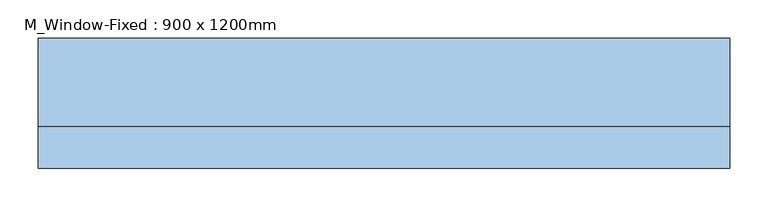
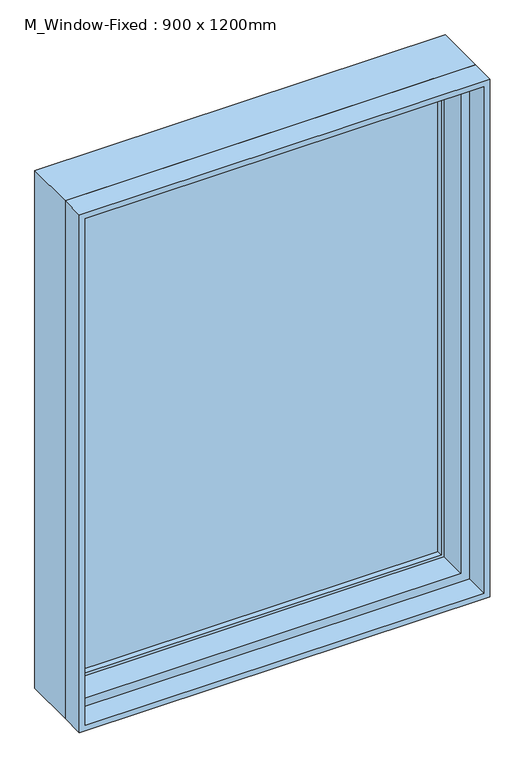
"""IFC4 building model written with IfcOpenShell, lengths in millimetres: window geometry, M_Window-Fixed : 900 x 1200mm."""

import ifcopenshell
import ifcopenshell.guid

model = None  # the IFC model being written
_history = None  # IfcOwnerHistory: only IFC2X3 demands one
_inside = {}  # id of a spatial element -> (the spatial element, [elements in it])
_under = {}  # id of a project, library or spatial element -> (it, [spatial elements below it])
_declared = {}  # id of a project -> (the project, [libraries it declares])
_typed = {}  # id of a type object -> (the type object, [elements of that type])
_made_of = {}  # id of a material, layer set ... -> (it, [elements and type objects made of it])


def new_model(schema):
    """Start an empty IFC model of exactly this schema.

    Asked for "IFC4X3", IfcOpenShell would pick the latest addendum, in which some entities
    have other attributes; the version numbers below select the first issue.
    IFC2X3 requires an IfcOwnerHistory on every rooted entity: one is made here for all.
    """
    global model, _history
    if schema == "IFC4X3":
        model = ifcopenshell.file(schema_version=(4, 3, 0, 0))
    else:
        model = ifcopenshell.file(schema=schema)
    _inside.clear()
    _under.clear()
    _declared.clear()
    _typed.clear()
    _made_of.clear()
    _history = None
    if model.schema == "IFC2X3":
        org = make("IfcOrganization", Name="unknown")
        user = make(
            "IfcPersonAndOrganization",
            ThePerson=make("IfcPerson", FamilyName="unknown"),
            TheOrganization=org,
        )
        app = make(
            "IfcApplication",
            ApplicationDeveloper=org,
            Version="unknown",
            ApplicationFullName="unknown",
            ApplicationIdentifier="unknown",
        )
        _history = make(
            "IfcOwnerHistory",
            OwningUser=user,
            OwningApplication=app,
            ChangeAction="ADDED",
            CreationDate=0,
        )
    return model


def make(cls, **values):
    """One entity of the class cls with the attributes given. An attribute that is None is left unset."""
    return model.create_entity(
        cls, **{name: value for name, value in values.items() if value is not None}
    )


def rooted(cls, **values):
    """An entity with a GlobalId (a new one), such as an element, a storey or a relation."""
    return make(cls, GlobalId=ifcopenshell.guid.new(), OwnerHistory=_history, **values)


def si_unit(unit_type, name, prefix=None):
    """IfcSIUnit, for example si_unit("LENGTHUNIT", "METRE", prefix="MILLI")."""
    return make("IfcSIUnit", UnitType=unit_type, Prefix=prefix, Name=name)


def assignment(units):
    """IfcUnitAssignment: the units of a project."""
    return None if units is None else make("IfcUnitAssignment", Units=units)


def point(xyz):
    """IfcCartesianPoint."""
    return None if xyz is None else make("IfcCartesianPoint", Coordinates=xyz)


def direction(xyz):
    """IfcDirection."""
    return None if xyz is None else make("IfcDirection", DirectionRatios=xyz)


def frame(location, z_axis=None, x_axis=None):
    """IfcAxis2Placement3D, a coordinate frame: its origin and axes. An axis left out is left unset."""
    return make(
        "IfcAxis2Placement3D",
        Location=point(location),
        Axis=direction(z_axis),
        RefDirection=direction(x_axis),
    )


def origin():
    """The frame at (0, 0, 0) with its axes left unset."""
    return frame((0.0, 0.0, 0.0))


def place(relative_to, where):
    """IfcLocalPlacement: puts the frame where relative to a parent placement (None: the world)."""
    return make(
        "IfcLocalPlacement", PlacementRelTo=relative_to, RelativePlacement=where
    )


def context(
    kind, dimensions, precision=None, world=None, true_north=None, identifier=None
):
    """IfcGeometricRepresentationContext, for example the 3D "Model" context."""
    return make(
        "IfcGeometricRepresentationContext",
        ContextIdentifier=identifier,
        ContextType=kind,
        CoordinateSpaceDimension=dimensions,
        Precision=precision,
        WorldCoordinateSystem=world,
        TrueNorth=true_north,
    )


def project(units=None, contexts=None):
    """IfcProject with its units and contexts."""
    return rooted(
        "IfcProject",
        Name="project",
        RepresentationContexts=contexts,
        UnitsInContext=assignment(units),
    )


def spatial(cls, under=None, at=None, **own):
    """A site, building, storey or space (cls), placed at a placement, below another one or the project."""
    s = rooted(cls, ObjectPlacement=at, **own)
    if under is not None:
        _under.setdefault(under.id(), (under, []))[1].append(s)
    return s


def polyline(points):
    """IfcPolyline through the points."""
    return make("IfcPolyline", Points=[point(p) for p in points])


def outline(outer, holes=None, kind="AREA"):
    """IfcArbitraryClosedProfileDef: a profile drawn as a closed curve; with holes, ...WithVoids."""
    if holes is None:
        return make("IfcArbitraryClosedProfileDef", ProfileType=kind, OuterCurve=outer)
    return make(
        "IfcArbitraryProfileDefWithVoids",
        ProfileType=kind,
        OuterCurve=outer,
        InnerCurves=holes,
    )


def extrude(swept, where, along, depth):
    """IfcExtrudedAreaSolid: the profile swept, set in the frame where, extruded along a direction by depth."""
    return make(
        "IfcExtrudedAreaSolid",
        SweptArea=swept,
        Position=where,
        ExtrudedDirection=direction(along),
        Depth=depth,
    )


def faces_of(points, faces, orient=None, outer=None):
    """IfcFace entities. A face is a list of loops; a loop is a list of indices into points, from 0.

    orient and outer hold one flag for each loop. By default every Orientation is true, the
    first loop of a face is its IfcFaceOuterBound and the others are IfcFaceBound.
    """
    made = []
    for i, loops in enumerate(faces):
        bounds = []
        for j, loop in enumerate(loops):
            is_outer = j == 0 if outer is None else outer[i][j]
            bounds.append(
                make(
                    "IfcFaceOuterBound" if is_outer else "IfcFaceBound",
                    Bound=make("IfcPolyLoop", Polygon=[points[k] for k in loop]),
                    Orientation=True if orient is None else orient[i][j],
                )
            )
        made.append(make("IfcFace", Bounds=bounds))
    return made


def faceted_brep(points, faces, orient=None, outer=None, voids=None):
    """IfcFacetedBrep: a solid bounded by flat faces; with voids (closed shells), ...WithVoids."""
    shared = [point(p) for p in points]
    hull = make("IfcClosedShell", CfsFaces=faces_of(shared, faces, orient, outer))
    if voids is None:
        return make("IfcFacetedBrep", Outer=hull)
    return make(
        "IfcFacetedBrepWithVoids",
        Outer=hull,
        Voids=[
            make(cls, CfsFaces=faces_of(shared, fs, o, b)) for cls, fs, o, b in voids
        ],
    )


def shape(context_of_items, identifier, shape_type, items):
    """IfcShapeRepresentation: the items that make up one representation, for example the "Body"."""
    return make(
        "IfcShapeRepresentation",
        ContextOfItems=context_of_items,
        RepresentationIdentifier=identifier,
        RepresentationType=shape_type,
        Items=items,
    )


def source(mapping_origin, context_of_items, identifier, shape_type, items):
    """IfcRepresentationMap: a shape defined once, which mapped items show again and again."""
    return make(
        "IfcRepresentationMap",
        MappingOrigin=mapping_origin,
        MappedRepresentation=shape(context_of_items, identifier, shape_type, items),
    )


def transform(
    local_origin,
    x_axis=None,
    y_axis=None,
    z_axis=None,
    scale=None,
    scale2=None,
    scale3=None,
    uniform=True,
):
    """IfcCartesianTransformationOperator3D, or its non-uniform kind. x_axis, y_axis, z_axis: its Axis1, 2, 3."""
    if uniform:
        return make(
            "IfcCartesianTransformationOperator3D",
            Axis1=direction(x_axis),
            Axis2=direction(y_axis),
            LocalOrigin=point(local_origin),
            Scale=scale,
            Axis3=direction(z_axis),
        )
    return make(
        "IfcCartesianTransformationOperator3DnonUniform",
        Axis1=direction(x_axis),
        Axis2=direction(y_axis),
        LocalOrigin=point(local_origin),
        Scale=scale,
        Axis3=direction(z_axis),
        Scale2=scale2,
        Scale3=scale3,
    )


def mapped(mapping_source, mapping_target):
    """IfcMappedItem: shows the shape of a source again, moved by a transform."""
    return make(
        "IfcMappedItem", MappingSource=mapping_source, MappingTarget=mapping_target
    )


def made_of(thing, what):
    """Note that an element or type object is made of a material, layer set ...; save() writes the relation."""
    if what is not None:
        _made_of.setdefault(what.id(), (what, []))[1].append(thing)
    return thing


def element(
    cls,
    number,
    at=None,
    inside=None,
    cuts=None,
    type_object=None,
    material=None,
    context=None,
    identifier="Body",
    shape_type=None,
    held_by="IfcProductDefinitionShape",
    body=None,
    shapes=None,
    **own,
):
    """One element of the class cls, such as IfcWall. Its Tag is "e" and its number.

    at: its placement. inside: the storey or other place that contains it. cuts: it is an
    opening in that element (IfcRelVoidsElement). A single representation is given by context,
    identifier, shape_type and body (its items); several are given by shapes. held_by: the class
    of the entity that holds the representations. save() writes the other relations.
    """
    e = rooted(cls, Tag="e%d" % number, ObjectPlacement=at, **own)
    if body is not None:
        shapes = [shape(context, identifier, shape_type, body)]
    if shapes is not None:
        e.Representation = make(held_by, Representations=shapes)
    if inside is not None:
        _inside.setdefault(inside.id(), (inside, []))[1].append(e)
    if cuts is not None:
        rooted(
            "IfcRelVoidsElement", RelatingBuildingElement=cuts, RelatedOpeningElement=e
        )
    if type_object is not None:
        _typed.setdefault(type_object.id(), (type_object, []))[1].append(e)
    return made_of(e, material)


def aggregate(whole, parts):
    """IfcRelAggregates: a whole, such as a stair, and the parts it consists of."""
    return rooted("IfcRelAggregates", RelatingObject=whole, RelatedObjects=parts)


def save(model, path):
    """Write the relations noted so far, then the file.

    IfcRelAggregates (storeys below a building ...), IfcRelContainedInSpatialStructure (elements
    in a storey), IfcRelDefinesByType, IfcRelAssociatesMaterial and IfcRelDeclares: one each for
    every whole, place, type object, material and project.
    """
    for whole, parts in _under.values():
        aggregate(whole, parts)
    for where, things in _inside.values():
        rooted(
            "IfcRelContainedInSpatialStructure",
            RelatedElements=things,
            RelatingStructure=where,
        )
    for kind, things in _typed.values():
        rooted("IfcRelDefinesByType", RelatedObjects=things, RelatingType=kind)
    for what, things in _made_of.values():
        rooted("IfcRelAssociatesMaterial", RelatedObjects=things, RelatingMaterial=what)
    for by, libraries in _declared.values():
        rooted("IfcRelDeclares", RelatingContext=by, RelatedDefinitions=libraries)
    model.write(path)


def m_window_fixed_900_x_1200mm_f2c8dc95(model_context):
    return source(origin(), model_context, "Body", "SolidModel", [
        faceted_brep([(450.0, -20.25, 2100.0), (450.0, 94.05, 2100.0), (-450.0, 94.05, 2100.0), (-450.0, -20.25, 2100.0), (-450.0, 94.05, 900.0), (-450.0, -20.25, 900.0), (450.0, 94.05, 900.0), (450.0, -20.25, 900.0), (418.25, -20.25, 2068.25), (418.25, -20.25, 931.75), (-418.25, -20.25, 931.75), (-418.25, -20.25, 2068.25), (-437.3, 94.05, 2087.3), (-437.3, 94.05, 912.7), (437.3, 94.05, 912.7), (437.3, 94.05, 2087.3), (418.25, 43.25, 2068.25), (-418.25, 43.25, 2068.25), (437.3, 43.25, 2087.3), (-437.3, 43.25, 2087.3), (-418.25, 43.25, 931.75), (-437.3, 43.25, 912.7), (418.25, 43.25, 931.75), (437.3, 43.25, 912.7)], [[[0, 1, 2, 3]], [[3, 2, 4, 5]], [[5, 4, 6, 7]], [[3, 5, 7, 0], [8, 9, 10, 11]], [[7, 6, 1, 0]], [[1, 6, 4, 2], [12, 13, 14, 15]], [[16, 8, 11, 17]], [[15, 18, 19, 12]], [[17, 11, 10, 20]], [[12, 19, 21, 13]], [[20, 10, 9, 22]], [[13, 21, 23, 14]], [[22, 9, 8, 16]], [[18, 23, 21, 19], [17, 20, 22, 16]], [[14, 23, 18, 15]]]),
        extrude(outline(polyline([(2100.0, -450.0), (900.0, -450.0), (900.0, 450.0), (2100.0, 450.0), (2100.0, -450.0)]), holes=[polyline([(2087.3, 437.3), (912.7, 437.3), (912.7, -437.3), (2087.3, -437.3), (2087.3, 437.3)])]), frame((0.0, -75.0, 0.0), z_axis=(0.0, 1.0, 0.0), x_axis=(0.0, 0.0, 1.0)), (0.0, 0.0, 1.0), 54.75),
        extrude(outline(polyline([(912.7, 437.3), (2087.3, 437.3), (2087.3, -437.3), (912.7, -437.3), (912.7, 437.3)]), holes=[polyline([(938.1, -411.9), (2061.9, -411.9), (2061.9, 411.9), (938.1, 411.9), (938.1, -411.9)])]), frame((0.0, 43.25, 0.0), z_axis=(0.0, 1.0, 0.0), x_axis=(0.0, 0.0, 1.0)), (0.0, 0.0, 1.0), 44.45),
        extrude(outline(polyline([(411.9, 75.0), (411.9, 68.65), (-411.9, 68.65), (-411.9, 75.0), (411.9, 75.0)])), frame((0.0, 0.0, 938.1), z_axis=(0.0, 0.0, 1.0), x_axis=(1.0, 0.0, 0.0)), (0.0, 0.0, 1.0), 1123.8),
        extrude(outline(polyline([(-411.9, 55.95), (-411.9, 62.3), (411.9, 62.3), (411.9, 55.95), (-411.9, 55.95)])), frame((0.0, 0.0, 938.1), z_axis=(0.0, 0.0, 1.0), x_axis=(1.0, 0.0, 0.0)), (0.0, 0.0, 1.0), 1123.8),
    ])


if __name__ == "__main__":
    model = new_model("IFC4")
    model_context = context("Model", 3, world=origin())
    ifc_project = project(units=[si_unit("LENGTHUNIT", "METRE", prefix="MILLI")], contexts=[model_context])
    site = spatial("IfcSite", under=ifc_project)
    building = spatial("IfcBuilding", under=site)
    placement = place(None, origin())
    m_window_fixed_900_x_1200mm_shape = m_window_fixed_900_x_1200mm_f2c8dc95(model_context)
    element("IfcWindow", 1, ObjectType="M_Window-Fixed : 900 x 1200mm", at=placement, inside=building, context=model_context, shape_type="MappedRepresentation", body=[
        mapped(m_window_fixed_900_x_1200mm_shape, transform((0.0, 0.0, 0.0), x_axis=(1.0, 0.0, 0.0), y_axis=(0.0, 1.0, 0.0), z_axis=(0.0, 0.0, 1.0))),
    ])
    save(model, "model.ifc")

# Revit data of these elements
# Type "M_Window-Fixed : 900 x 1200mm"
#   Type Mark = "36"
#   Fire Rating = "0.5h"
#   Analytic Construction = "Double glazing - domestic"
#   Window Inset [instance default] = 0 mm
#   Wall Thickness [instance default] = 150 mm
#   Visual Light Transmittance = 0.81
#   Thermal Resistance (R) = 0.319569 (m²·K)/W
#   Solar Heat Gain Coefficient = 0.76
#   Rough Width = 915 mm
#   Rough Height = 1215 mm
#   Interior Wall Closure [instance default] = 54.75 mm
#   Height = 1200 mm
#   Heat Transfer Coefficient (U) = 3.12929 W/(m²·K)
#   Frame Extension [instance default] = 6.35 mm
#   Exterior Wall Closure [instance default] = 31.75 mm
#   Extension Jamb [instance default] = 54.75 mm
#   Default Sill Height = 900 mm
#   Width = 900 mm
#   Muntin Visibility = yes
#   Interior Trim Visibility [instance default] = yes
#   Exterior Trim Visibility [instance default] = yes
#   Extension Jamb Visibility [instance default] = yes
#   Muntin Pattern = M_Muntin Pattern_2x2 : M_Muntin Pattern_2x2
#   Interior Trim Material = Wood - Stained
#   Interior Trim = M_Trim-Window-Interior-Flat : Picture Frame
#   Interior Frame Material = Wood - Stained
#   Glass Panel Material = Glass
#   Exterior Trim Material = Clad - White
#   Exterior Trim = M_Trim-Window-Exterior-Flat : with Sill
#   Exterior Frame Material = Clad - White
#   Wall Closure = (empty or 0)
# Element 1 (IfcWindow, "M_Window-Fixed : 900 x 1200mm")
#   Materials on its faces: "Wood - Stained", "Glass", "Clad - White"
# Materials
#   "Wood - Stained": class "Wood", colour RGB 173 132 96, transparency 0, Cost = 0
#   "Glass": class "Glass", colour RGB 245 245 243, transparency 1, Description = "Soda Lime Glass", Cost = 0
#   "Clad - White": class "Wood", colour RGB 245 245 243, transparency 0, Cost = 0
